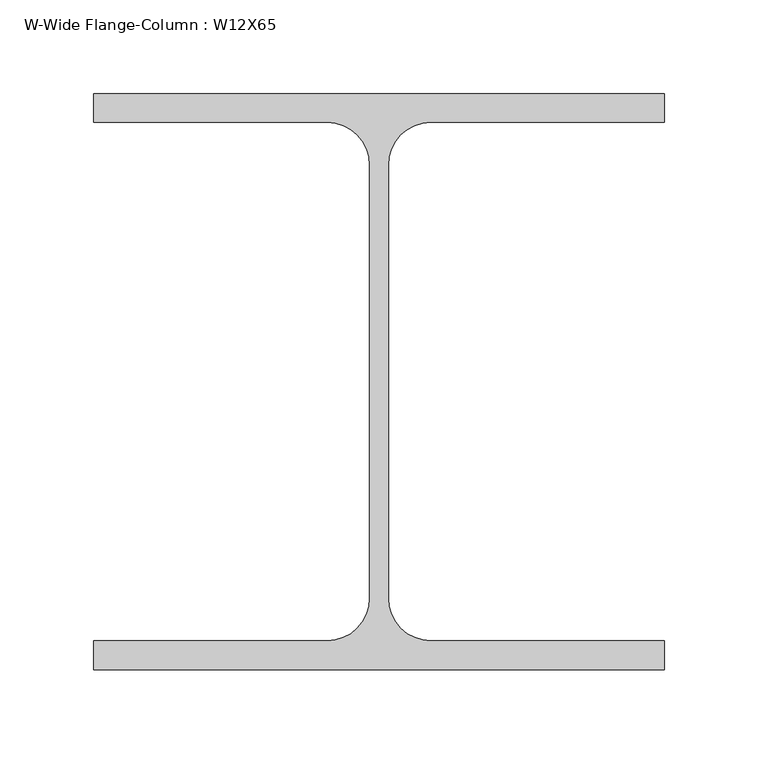
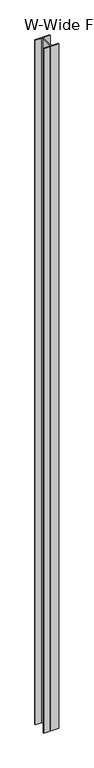
"""IFC4 building model written with IfcOpenShell, lengths in millimetres: column geometry, W-Wide Flange-Column : W12X65."""

from ifc_helpers import new_model, si_unit, point, frame, frame_2d, origin, place, context, project, spatial, polyline, circle_curve, trimmed, segment, composite_curve, outline, extrude, source, transform, mapped, element, save


def w_wide_flange_column_w12x65_9297464c(model_context):
    return source(origin(), model_context, "Body", "SweptSolid", [
        extrude(outline(composite_curve([segment(polyline([(152.4, 153.67), (152.4, 138.303), (27.686, 138.303)]), True, "CONTINUOUS"), segment(trimmed(circle_curve(frame_2d((27.686, 115.57)), 22.733), [point((27.686, 138.303))], [point((4.953, 115.57))], True, "CARTESIAN"), True, "CONTINUOUS"), segment(polyline([(4.953, 115.57), (4.953, -115.57)]), True, "CONTINUOUS"), segment(trimmed(circle_curve(frame_2d((27.686, -115.57)), 22.733), [point((4.953, -115.57))], [point((27.686, -138.303))], True, "CARTESIAN"), True, "CONTINUOUS"), segment(polyline([(27.686, -138.303), (152.4, -138.303), (152.4, -153.67), (-152.4, -153.67), (-152.4, -138.303), (-27.686, -138.303)]), True, "CONTINUOUS"), segment(trimmed(circle_curve(frame_2d((-27.686, -115.57)), 22.733), [point((-27.686, -138.303))], [point((-4.953, -115.57))], True, "CARTESIAN"), True, "CONTINUOUS"), segment(polyline([(-4.953, -115.57), (-4.953, 115.57)]), True, "CONTINUOUS"), segment(trimmed(circle_curve(frame_2d((-27.686, 115.57)), 22.733), [point((-4.953, 115.57))], [point((-27.686, 138.303))], True, "CARTESIAN"), True, "CONTINUOUS"), segment(polyline([(-27.686, 138.303), (-152.4, 138.303), (-152.4, 153.67), (152.4, 153.67)]), True, "CONTINUOUS")], self_intersect=False)), frame((0.0, 0.0, 8655.05), z_axis=(0.0, 0.0, 1.0), x_axis=(1.0, 0.0, 0.0)), (0.0, 0.0, 1.0), 14662.15),
    ])


if __name__ == "__main__":
    model = new_model("IFC4")
    model_context = context("Model", 3, world=origin())
    ifc_project = project(units=[si_unit("LENGTHUNIT", "METRE", prefix="MILLI")], contexts=[model_context])
    site = spatial("IfcSite", under=ifc_project)
    building = spatial("IfcBuilding", under=site)
    placement = place(None, origin())
    w_wide_flange_column_w12x65_shape = w_wide_flange_column_w12x65_9297464c(model_context)
    element("IfcColumn", 1, ObjectType="W-Wide Flange-Column : W12X65", at=placement, inside=building, context=model_context, shape_type="MappedRepresentation", body=[
        mapped(w_wide_flange_column_w12x65_shape, transform((0.0, 0.0, 0.0), x_axis=(1.0, 0.0, 0.0), y_axis=(0.0, 1.0, 0.0), z_axis=(0.0, 0.0, 1.0))),
    ])
    save(model, "model.ifc")

# Revit data of these elements
# Type "W-Wide Flange-Column : W12X65"
#   Assembly Code = "B10"
#   W = 65
#   bf = 1' - 0"
#   d = 1' - 0.1"
#   k = 0' - 1 1/2"
#   kr = 0' - 0.895"
#   tf = 0' - 0.605"
#   tw = 0' - 0.39"
#   A = 0.132639 SF
#   Structural Material [instance default] = Steel ASTM A992
# Element 1 (IfcColumn, "W-Wide Flange-Column : W12X65")
#   Materials on its faces: "Steel ASTM A992"
# Materials
#   "Steel ASTM A992": class "Metal", colour RGB 199 199 199, transparency 0, Description = "Structural steel 50ksi", Cost = 0
